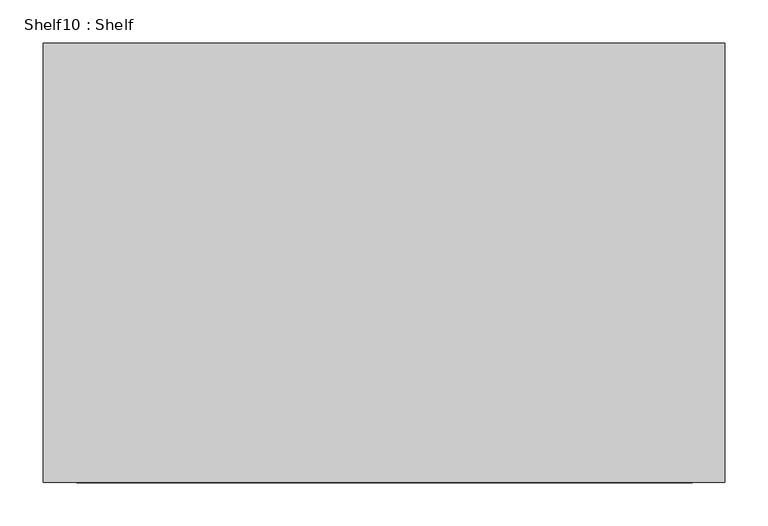
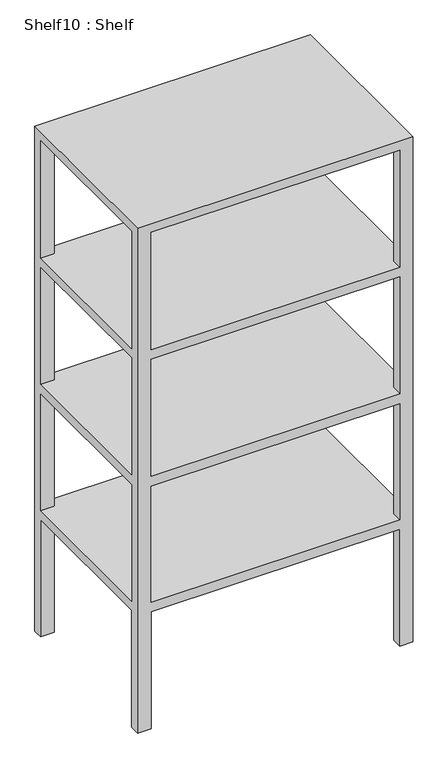
"""IFC4 building model written with IfcOpenShell, lengths in millimetres: furniture geometry, Shelf10 : Shelf."""

import ifcopenshell
import ifcopenshell.guid

model = None  # the IFC model being written
_history = None  # IfcOwnerHistory: only IFC2X3 demands one
_inside = {}  # id of a spatial element -> (the spatial element, [elements in it])
_under = {}  # id of a project, library or spatial element -> (it, [spatial elements below it])
_declared = {}  # id of a project -> (the project, [libraries it declares])
_typed = {}  # id of a type object -> (the type object, [elements of that type])
_made_of = {}  # id of a material, layer set ... -> (it, [elements and type objects made of it])


def new_model(schema):
    """Start an empty IFC model of exactly this schema.

    Asked for "IFC4X3", IfcOpenShell would pick the latest addendum, in which some entities
    have other attributes; the version numbers below select the first issue.
    IFC2X3 requires an IfcOwnerHistory on every rooted entity: one is made here for all.
    """
    global model, _history
    if schema == "IFC4X3":
        model = ifcopenshell.file(schema_version=(4, 3, 0, 0))
    else:
        model = ifcopenshell.file(schema=schema)
    _inside.clear()
    _under.clear()
    _declared.clear()
    _typed.clear()
    _made_of.clear()
    _history = None
    if model.schema == "IFC2X3":
        org = make("IfcOrganization", Name="unknown")
        user = make(
            "IfcPersonAndOrganization",
            ThePerson=make("IfcPerson", FamilyName="unknown"),
            TheOrganization=org,
        )
        app = make(
            "IfcApplication",
            ApplicationDeveloper=org,
            Version="unknown",
            ApplicationFullName="unknown",
            ApplicationIdentifier="unknown",
        )
        _history = make(
            "IfcOwnerHistory",
            OwningUser=user,
            OwningApplication=app,
            ChangeAction="ADDED",
            CreationDate=0,
        )
    return model


def make(cls, **values):
    """One entity of the class cls with the attributes given. An attribute that is None is left unset."""
    return model.create_entity(
        cls, **{name: value for name, value in values.items() if value is not None}
    )


def rooted(cls, **values):
    """An entity with a GlobalId (a new one), such as an element, a storey or a relation."""
    return make(cls, GlobalId=ifcopenshell.guid.new(), OwnerHistory=_history, **values)


def si_unit(unit_type, name, prefix=None):
    """IfcSIUnit, for example si_unit("LENGTHUNIT", "METRE", prefix="MILLI")."""
    return make("IfcSIUnit", UnitType=unit_type, Prefix=prefix, Name=name)


def assignment(units):
    """IfcUnitAssignment: the units of a project."""
    return None if units is None else make("IfcUnitAssignment", Units=units)


def point(xyz):
    """IfcCartesianPoint."""
    return None if xyz is None else make("IfcCartesianPoint", Coordinates=xyz)


def direction(xyz):
    """IfcDirection."""
    return None if xyz is None else make("IfcDirection", DirectionRatios=xyz)


def frame(location, z_axis=None, x_axis=None):
    """IfcAxis2Placement3D, a coordinate frame: its origin and axes. An axis left out is left unset."""
    return make(
        "IfcAxis2Placement3D",
        Location=point(location),
        Axis=direction(z_axis),
        RefDirection=direction(x_axis),
    )


def origin():
    """The frame at (0, 0, 0) with its axes left unset."""
    return frame((0.0, 0.0, 0.0))


def place(relative_to, where):
    """IfcLocalPlacement: puts the frame where relative to a parent placement (None: the world)."""
    return make(
        "IfcLocalPlacement", PlacementRelTo=relative_to, RelativePlacement=where
    )


def context(
    kind, dimensions, precision=None, world=None, true_north=None, identifier=None
):
    """IfcGeometricRepresentationContext, for example the 3D "Model" context."""
    return make(
        "IfcGeometricRepresentationContext",
        ContextIdentifier=identifier,
        ContextType=kind,
        CoordinateSpaceDimension=dimensions,
        Precision=precision,
        WorldCoordinateSystem=world,
        TrueNorth=true_north,
    )


def project(units=None, contexts=None):
    """IfcProject with its units and contexts."""
    return rooted(
        "IfcProject",
        Name="project",
        RepresentationContexts=contexts,
        UnitsInContext=assignment(units),
    )


def spatial(cls, under=None, at=None, **own):
    """A site, building, storey or space (cls), placed at a placement, below another one or the project."""
    s = rooted(cls, ObjectPlacement=at, **own)
    if under is not None:
        _under.setdefault(under.id(), (under, []))[1].append(s)
    return s


def faces_of(points, faces, orient=None, outer=None):
    """IfcFace entities. A face is a list of loops; a loop is a list of indices into points, from 0.

    orient and outer hold one flag for each loop. By default every Orientation is true, the
    first loop of a face is its IfcFaceOuterBound and the others are IfcFaceBound.
    """
    made = []
    for i, loops in enumerate(faces):
        bounds = []
        for j, loop in enumerate(loops):
            is_outer = j == 0 if outer is None else outer[i][j]
            bounds.append(
                make(
                    "IfcFaceOuterBound" if is_outer else "IfcFaceBound",
                    Bound=make("IfcPolyLoop", Polygon=[points[k] for k in loop]),
                    Orientation=True if orient is None else orient[i][j],
                )
            )
        made.append(make("IfcFace", Bounds=bounds))
    return made


def faceted_brep(points, faces, orient=None, outer=None, voids=None):
    """IfcFacetedBrep: a solid bounded by flat faces; with voids (closed shells), ...WithVoids."""
    shared = [point(p) for p in points]
    hull = make("IfcClosedShell", CfsFaces=faces_of(shared, faces, orient, outer))
    if voids is None:
        return make("IfcFacetedBrep", Outer=hull)
    return make(
        "IfcFacetedBrepWithVoids",
        Outer=hull,
        Voids=[
            make(cls, CfsFaces=faces_of(shared, fs, o, b)) for cls, fs, o, b in voids
        ],
    )


def shape(context_of_items, identifier, shape_type, items):
    """IfcShapeRepresentation: the items that make up one representation, for example the "Body"."""
    return make(
        "IfcShapeRepresentation",
        ContextOfItems=context_of_items,
        RepresentationIdentifier=identifier,
        RepresentationType=shape_type,
        Items=items,
    )


def source(mapping_origin, context_of_items, identifier, shape_type, items):
    """IfcRepresentationMap: a shape defined once, which mapped items show again and again."""
    return make(
        "IfcRepresentationMap",
        MappingOrigin=mapping_origin,
        MappedRepresentation=shape(context_of_items, identifier, shape_type, items),
    )


def transform(
    local_origin,
    x_axis=None,
    y_axis=None,
    z_axis=None,
    scale=None,
    scale2=None,
    scale3=None,
    uniform=True,
):
    """IfcCartesianTransformationOperator3D, or its non-uniform kind. x_axis, y_axis, z_axis: its Axis1, 2, 3."""
    if uniform:
        return make(
            "IfcCartesianTransformationOperator3D",
            Axis1=direction(x_axis),
            Axis2=direction(y_axis),
            LocalOrigin=point(local_origin),
            Scale=scale,
            Axis3=direction(z_axis),
        )
    return make(
        "IfcCartesianTransformationOperator3DnonUniform",
        Axis1=direction(x_axis),
        Axis2=direction(y_axis),
        LocalOrigin=point(local_origin),
        Scale=scale,
        Axis3=direction(z_axis),
        Scale2=scale2,
        Scale3=scale3,
    )


def mapped(mapping_source, mapping_target):
    """IfcMappedItem: shows the shape of a source again, moved by a transform."""
    return make(
        "IfcMappedItem", MappingSource=mapping_source, MappingTarget=mapping_target
    )


def made_of(thing, what):
    """Note that an element or type object is made of a material, layer set ...; save() writes the relation."""
    if what is not None:
        _made_of.setdefault(what.id(), (what, []))[1].append(thing)
    return thing


def element(
    cls,
    number,
    at=None,
    inside=None,
    cuts=None,
    type_object=None,
    material=None,
    context=None,
    identifier="Body",
    shape_type=None,
    held_by="IfcProductDefinitionShape",
    body=None,
    shapes=None,
    **own,
):
    """One element of the class cls, such as IfcWall. Its Tag is "e" and its number.

    at: its placement. inside: the storey or other place that contains it. cuts: it is an
    opening in that element (IfcRelVoidsElement). A single representation is given by context,
    identifier, shape_type and body (its items); several are given by shapes. held_by: the class
    of the entity that holds the representations. save() writes the other relations.
    """
    e = rooted(cls, Tag="e%d" % number, ObjectPlacement=at, **own)
    if body is not None:
        shapes = [shape(context, identifier, shape_type, body)]
    if shapes is not None:
        e.Representation = make(held_by, Representations=shapes)
    if inside is not None:
        _inside.setdefault(inside.id(), (inside, []))[1].append(e)
    if cuts is not None:
        rooted(
            "IfcRelVoidsElement", RelatingBuildingElement=cuts, RelatedOpeningElement=e
        )
    if type_object is not None:
        _typed.setdefault(type_object.id(), (type_object, []))[1].append(e)
    return made_of(e, material)


def aggregate(whole, parts):
    """IfcRelAggregates: a whole, such as a stair, and the parts it consists of."""
    return rooted("IfcRelAggregates", RelatingObject=whole, RelatedObjects=parts)


def save(model, path):
    """Write the relations noted so far, then the file.

    IfcRelAggregates (storeys below a building ...), IfcRelContainedInSpatialStructure (elements
    in a storey), IfcRelDefinesByType, IfcRelAssociatesMaterial and IfcRelDeclares: one each for
    every whole, place, type object, material and project.
    """
    for whole, parts in _under.values():
        aggregate(whole, parts)
    for where, things in _inside.values():
        rooted(
            "IfcRelContainedInSpatialStructure",
            RelatedElements=things,
            RelatingStructure=where,
        )
    for kind, things in _typed.values():
        rooted("IfcRelDefinesByType", RelatedObjects=things, RelatingType=kind)
    for what, things in _made_of.values():
        rooted("IfcRelAssociatesMaterial", RelatedObjects=things, RelatingMaterial=what)
    for by, libraries in _declared.values():
        rooted("IfcRelDeclares", RelatingContext=by, RelatedDefinitions=libraries)
    model.write(path)


def shelf10_shelf_7f4ece80(model_context):
    return source(origin(), model_context, "Body", "Brep", [
        faceted_brep([(14906.8798744, 2223.7615366, 1524.0), (14906.8798744, 2731.7615366, 1524.0), (14119.4798744, 2731.7615366, 1524.0), (14119.4798744, 2223.7615366, 1524.0), (14906.8798744, 2223.7615366, 0.0), (14869.5001442, 2223.7615366, 0.0), (14869.5001442, 2252.7838057, 0.0), (14906.8798744, 2252.7838057, 0.0), (14869.5001442, 2731.7615366, 0.0), (14906.8798744, 2731.7615366, 0.0), (14906.8798744, 2702.8377422, 0.0), (14869.5001442, 2702.8377422, 0.0), (14158.3001442, 2223.7615366, 0.0), (14119.4798744, 2223.7615366, 0.0), (14119.4798744, 2252.7838057, 0.0), (14158.3001442, 2252.7838057, 0.0), (14119.4798744, 2702.8377422, 0.0), (14119.4798744, 2731.7615366, 0.0), (14158.3001442, 2731.7615366, 0.0), (14158.3001442, 2702.8377422, 0.0), (14158.3001442, 2223.7615366, 353.3332002), (14869.5001442, 2223.7615366, 353.3332002), (14158.3001442, 2223.7615366, 1497.6781444), (14869.5001442, 2223.7615366, 1497.6781444), (14869.5001442, 2223.7615366, 1143.0), (14158.3001442, 2223.7615366, 1143.0), (14158.3001442, 2223.7615366, 1114.8196695), (14869.5001442, 2223.7615366, 1114.8196695), (14869.5001442, 2223.7615366, 762.0), (14158.3001442, 2223.7615366, 762.0), (14158.3001442, 2223.7615366, 731.9611947), (14869.5001442, 2223.7615366, 731.9611947), (14869.5001442, 2223.7615366, 381.0), (14158.3001442, 2223.7615366, 381.0), (14119.4798744, 2702.8377422, 353.3332002), (14119.4798744, 2252.7838057, 353.3332002), (14119.4798744, 2702.8377422, 1497.6781444), (14119.4798744, 2252.3559348, 1497.6781444), (14119.4798744, 2252.3559348, 1143.0), (14119.4798744, 2702.8377422, 1143.0), (14119.4798744, 2702.8377422, 1114.8196695), (14119.4798744, 2252.7838057, 1114.8196695), (14119.4798744, 2252.7838057, 762.0), (14119.4798744, 2702.8377422, 762.0), (14119.4798744, 2702.8377422, 731.9611947), (14119.4798744, 2252.7838057, 731.9611947), (14119.4798744, 2252.7838057, 381.0), (14119.4798744, 2702.8377422, 381.0), (14869.5001442, 2731.7615366, 353.3332002), (14158.3001442, 2731.7615366, 353.3332002), (14869.5001442, 2731.7615366, 1497.6781444), (14158.3001442, 2731.7615366, 1497.6781444), (14158.3001442, 2731.7615366, 1143.0), (14869.5001442, 2731.7615366, 1143.0), (14869.5001442, 2731.7615366, 1114.8196695), (14158.3001442, 2731.7615366, 1114.8196695), (14158.3001442, 2731.7615366, 762.0), (14869.5001442, 2731.7615366, 762.0), (14869.5001442, 2731.7615366, 731.9611947), (14158.3001442, 2731.7615366, 731.9611947), (14158.3001442, 2731.7615366, 381.0), (14869.5001442, 2731.7615366, 381.0), (14906.8798744, 2252.7838057, 353.3332002), (14906.8798744, 2702.8377422, 353.3332002), (14906.8798744, 2252.7838057, 1497.6781444), (14906.8798744, 2702.8377422, 1497.6781444), (14906.8798744, 2702.8377422, 1143.0), (14906.8798744, 2252.7838057, 1143.0), (14906.8798744, 2252.7838057, 1114.8196695), (14906.8798744, 2702.8377422, 1114.8196695), (14906.8798744, 2702.8377422, 762.0), (14906.8798744, 2252.7838057, 762.0), (14906.8798744, 2252.7838057, 731.9611947), (14906.8798744, 2702.8377422, 731.9611947), (14906.8798744, 2702.8377422, 381.0), (14906.8798744, 2252.7838057, 381.0), (14158.3001442, 2702.8377422, 1497.6781444), (14869.5001442, 2702.8377422, 1497.6781444), (14869.5001442, 2252.7838057, 1497.6781444), (14158.3001442, 2252.3559348, 1497.6781444), (14158.3001442, 2702.8377422, 1143.0), (14158.3001442, 2252.3559348, 1143.0), (14869.5001442, 2252.7838057, 1143.0), (14869.5001442, 2702.8377422, 1143.0), (14158.3001442, 2702.8377422, 1114.8196695), (14869.5001442, 2702.8377422, 1114.8196695), (14869.5001442, 2252.7838057, 1114.8196695), (14158.3001442, 2252.7838057, 1114.8196695), (14158.3001442, 2702.8377422, 762.0), (14158.3001442, 2252.7838057, 762.0), (14869.5001442, 2252.7838057, 762.0), (14869.5001442, 2702.8377422, 762.0), (14158.3001442, 2702.8377422, 731.9611947), (14869.5001442, 2702.8377422, 731.9611947), (14869.5001442, 2252.7838057, 731.9611947), (14158.3001442, 2252.7838057, 731.9611947), (14158.3001442, 2702.8377422, 381.0), (14158.3001442, 2252.7838057, 381.0), (14869.5001442, 2252.7838057, 381.0), (14869.5001442, 2702.8377422, 381.0), (14158.3001442, 2702.8377422, 353.3332002), (14869.5001442, 2702.8377422, 353.3332002), (14869.5001442, 2252.7838057, 353.3332002), (14158.3001442, 2252.7838057, 353.3332002)], [[[0, 1, 2, 3]], [[4, 5, 6, 7]], [[8, 9, 10, 11]], [[12, 13, 14, 15]], [[16, 17, 18, 19]], [[0, 3, 13, 12, 20, 21, 5, 4], [22, 23, 24, 25], [26, 27, 28, 29], [30, 31, 32, 33]], [[3, 2, 17, 16, 34, 35, 14, 13], [36, 37, 38, 39], [40, 41, 42, 43], [44, 45, 46, 47]], [[2, 1, 9, 8, 48, 49, 18, 17], [50, 51, 52, 53], [54, 55, 56, 57], [58, 59, 60, 61]], [[1, 0, 4, 7, 62, 63, 10, 9], [64, 65, 66, 67], [68, 69, 70, 71], [72, 73, 74, 75]], [[76, 51, 50, 77, 65, 64, 78, 23, 22, 79, 37, 36]], [[80, 39, 38, 81, 25, 24, 82, 67, 66, 83, 53, 52]], [[51, 76, 80, 52]], [[77, 50, 53, 83]], [[65, 77, 83, 66]], [[78, 64, 67, 82]], [[23, 78, 82, 24]], [[79, 22, 25, 81]], [[37, 79, 81, 38]], [[76, 36, 39, 80]], [[84, 55, 54, 85, 69, 68, 86, 27, 26, 87, 41, 40]], [[88, 43, 42, 89, 29, 28, 90, 71, 70, 91, 57, 56]], [[55, 84, 88, 56]], [[85, 54, 57, 91]], [[69, 85, 91, 70]], [[86, 68, 71, 90]], [[27, 86, 90, 28]], [[87, 26, 29, 89]], [[41, 87, 89, 42]], [[84, 40, 43, 88]], [[92, 59, 58, 93, 73, 72, 94, 31, 30, 95, 45, 44]], [[96, 47, 46, 97, 33, 32, 98, 75, 74, 99, 61, 60]], [[59, 92, 96, 60]], [[93, 58, 61, 99]], [[73, 93, 99, 74]], [[94, 72, 75, 98]], [[31, 94, 98, 32]], [[95, 30, 33, 97]], [[45, 95, 97, 46]], [[92, 44, 47, 96]], [[100, 49, 48, 101, 63, 62, 102, 21, 20, 103, 35, 34]], [[49, 100, 19, 18]], [[101, 48, 8, 11]], [[63, 101, 11, 10]], [[102, 62, 7, 6]], [[21, 102, 6, 5]], [[103, 20, 12, 15]], [[35, 103, 15, 14]], [[100, 34, 16, 19]]]),
    ])


if __name__ == "__main__":
    model = new_model("IFC4")
    model_context = context("Model", 3, world=origin())
    ifc_project = project(units=[si_unit("LENGTHUNIT", "METRE", prefix="MILLI")], contexts=[model_context])
    site = spatial("IfcSite", under=ifc_project)
    building = spatial("IfcBuilding", under=site)
    placement = place(None, origin())
    shelf10_shelf_shape = shelf10_shelf_7f4ece80(model_context)
    element("IfcFurniture", 1, ObjectType="Shelf10 : Shelf", at=placement, inside=building, context=model_context, shape_type="MappedRepresentation", body=[
        mapped(shelf10_shelf_shape, transform((0.0, 0.0, 0.0), x_axis=(1.0, 0.0, 0.0), y_axis=(0.0, 1.0, 0.0), z_axis=(0.0, 0.0, 1.0))),
    ])
    save(model, "model.ifc")

# Revit data of these elements
# Element 1 (IfcFurniture, "Shelf10 : Shelf")
#   Materials on its faces: "food"
# Materials
#   "food": class "Glass", colour RGB 233 233 233, transparency 0, Description = "Soda Lime Glass", Cost = 0
